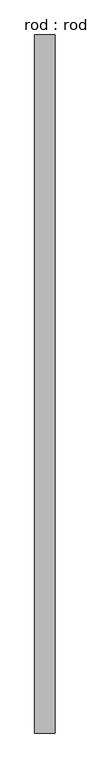
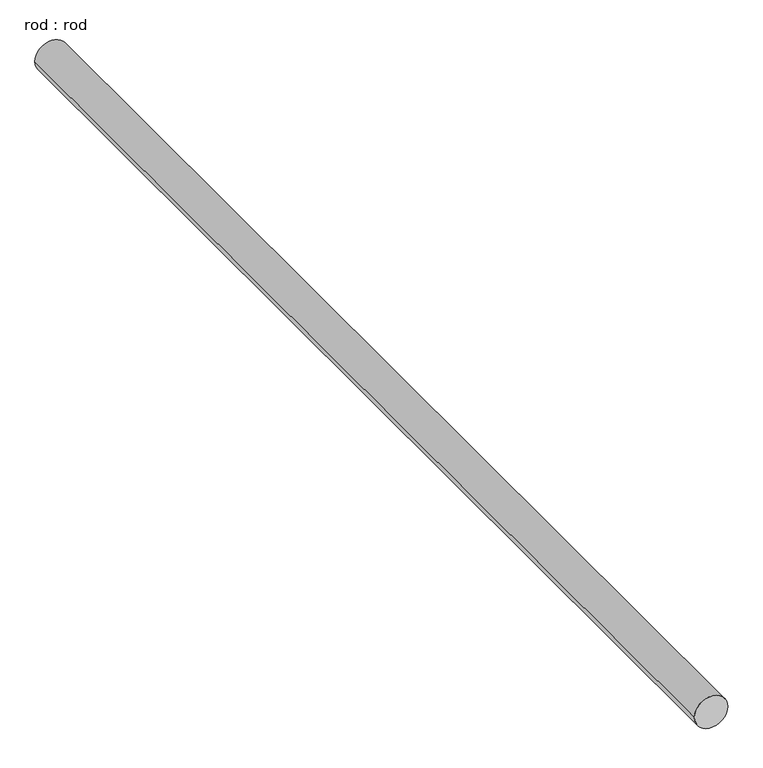
"""IFC4 building model written with IfcOpenShell, lengths in millimetres: proxy geometry, rod : rod."""

from ifc_helpers import new_model, si_unit, point, frame, frame_2d, origin, place, context, project, spatial, circle_curve, trimmed, segment, composite_curve, outline, extrude, source, transform, mapped, element, save


def rod_rod_93561386(model_context):
    return source(origin(), model_context, "Body", "SweptSolid", [
        extrude(outline(composite_curve([segment(trimmed(circle_curve(frame_2d((0.0108462, 0.0)), 200.0), [point((0.0108462, 200.0))], [point((0.0108462, -200.0))], False, "CARTESIAN"), True, "CONTINUOUS"), segment(trimmed(circle_curve(frame_2d((0.0108462, 0.0)), 200.0), [point((0.0108462, -200.0))], [point((0.0108462, 200.0))], False, "CARTESIAN"), True, "CONTINUOUS")], self_intersect=False)), frame((0.0, -2791.1999561, 0.0), z_axis=(0.0, 1.0, 0.0), x_axis=(0.0, 0.0, 1.0)), (0.0, 0.0, 1.0), 13767.8571429),
    ])


if __name__ == "__main__":
    model = new_model("IFC4")
    model_context = context("Model", 3, world=origin())
    ifc_project = project(units=[si_unit("LENGTHUNIT", "METRE", prefix="MILLI")], contexts=[model_context])
    site = spatial("IfcSite", under=ifc_project)
    building = spatial("IfcBuilding", under=site)
    placement = place(None, origin())
    rod_rod_shape = rod_rod_93561386(model_context)
    element("IfcBuildingElementProxy", 1, Name="rod : rod", ObjectType="rod : rod", at=placement, inside=building, context=model_context, shape_type="MappedRepresentation", body=[
        mapped(rod_rod_shape, transform((0.0, 0.0, 0.0), x_axis=(1.0, 0.0, 0.0), y_axis=(0.0, 1.0, 0.0), z_axis=(0.0, 0.0, 1.0))),
    ])
    save(model, "model.ifc")

# Revit data of these elements
# Type "rod : rod"
#   Default Elevation = 0
